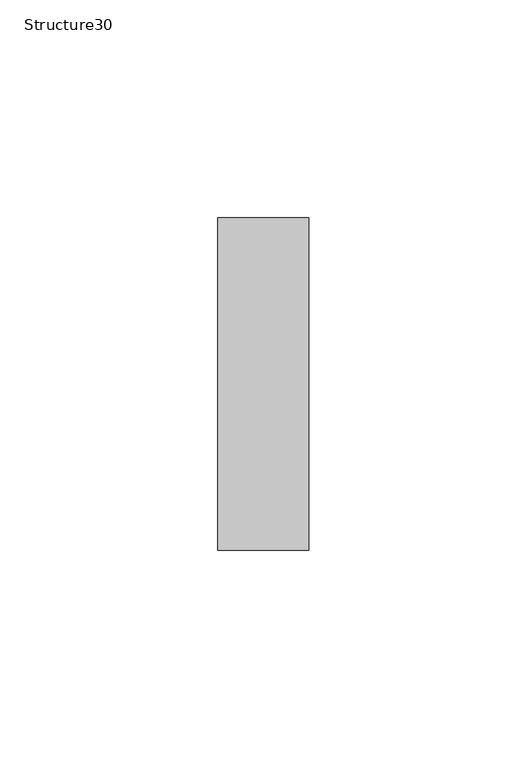
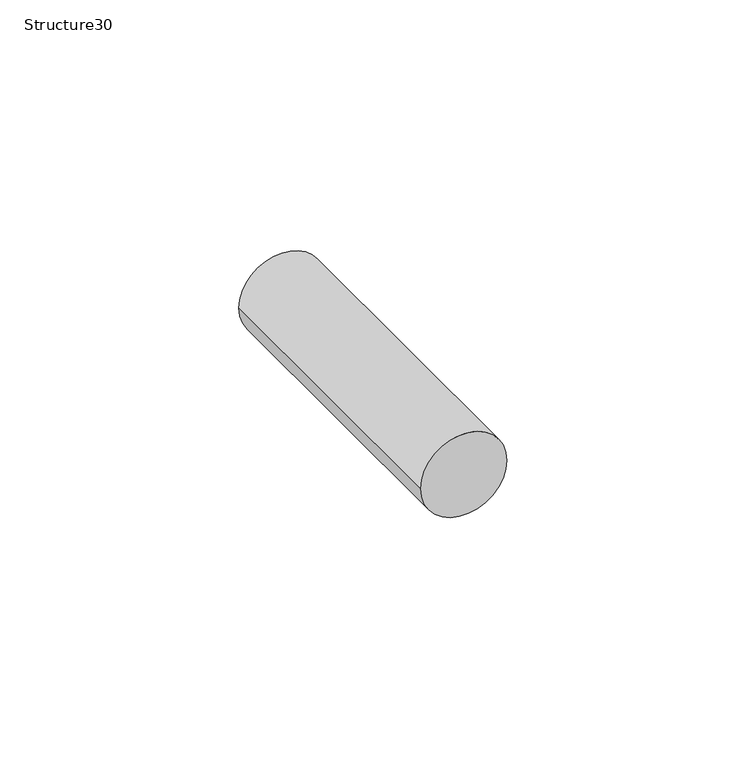
"""IFC4 building model written with IfcOpenShell, lengths in millimetres: proxy geometry, Structure30 : Structure668217128."""

from ifc_helpers import new_model, si_unit, point, frame, frame_2d, origin, place, context, project, spatial, circle_curve, trimmed, segment, composite_curve, outline, extrude, source, transform, mapped, element, save


def structure30_b6a8441b(model_context):
    return source(origin(), model_context, "Body", "SweptSolid", [
        extrude(outline(composite_curve([segment(trimmed(circle_curve(frame_2d((38047.8454063, 5185.7383658)), 10.4009751), [point((38047.8454063, 5175.3373907))], [point((38047.8454063, 5196.139341))], False, "CARTESIAN"), True, "CONTINUOUS"), segment(trimmed(circle_curve(frame_2d((38047.8454063, 5185.7383658)), 10.4009751), [point((38047.8454063, 5196.139341))], [point((38047.8454063, 5175.3373907))], False, "CARTESIAN"), True, "CONTINUOUS")], self_intersect=False)), frame((0.0, 935.5510696, 0.0), z_axis=(0.0, 1.0, 0.0), x_axis=(0.0, 0.0, 1.0)), (0.0, 0.0, 1.0), 76.2),
    ])


if __name__ == "__main__":
    model = new_model("IFC4")
    model_context = context("Model", 3, world=origin())
    ifc_project = project(units=[si_unit("LENGTHUNIT", "METRE", prefix="MILLI")], contexts=[model_context])
    site = spatial("IfcSite", under=ifc_project)
    building = spatial("IfcBuilding", under=site)
    placement = place(None, origin())
    structure30_shape = structure30_b6a8441b(model_context)
    element("IfcBuildingElementProxy", 1, Name="Structure30 : Structure668217128", ObjectType="Structure30 : Structure668217128", at=placement, inside=building, context=model_context, shape_type="MappedRepresentation", body=[
        mapped(structure30_shape, transform((0.0, 0.0, 0.0), x_axis=(1.0, 0.0, 0.0), y_axis=(0.0, 1.0, 0.0), z_axis=(0.0, 0.0, 1.0))),
    ])
    save(model, "model.ifc")

# Revit data of these elements
# Type "Structure30 : Structure668217128"
#   NameOverride = "Structure668217128"
# Element 1 (IfcBuildingElementProxy, "Structure30 : Structure668217128")
#   Materials on its faces: "1.5\" DIA. STAINLESS STEEL RAILING"
# Materials
#   "1.5\" DIA. STAINLESS STEEL RAILING": class "Unassigned", colour RGB 128 128 128, transparency 0, Cost = 0
